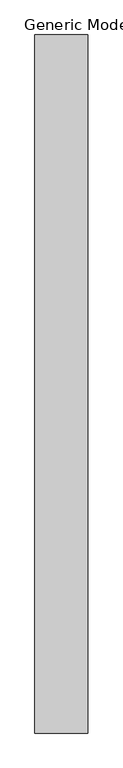
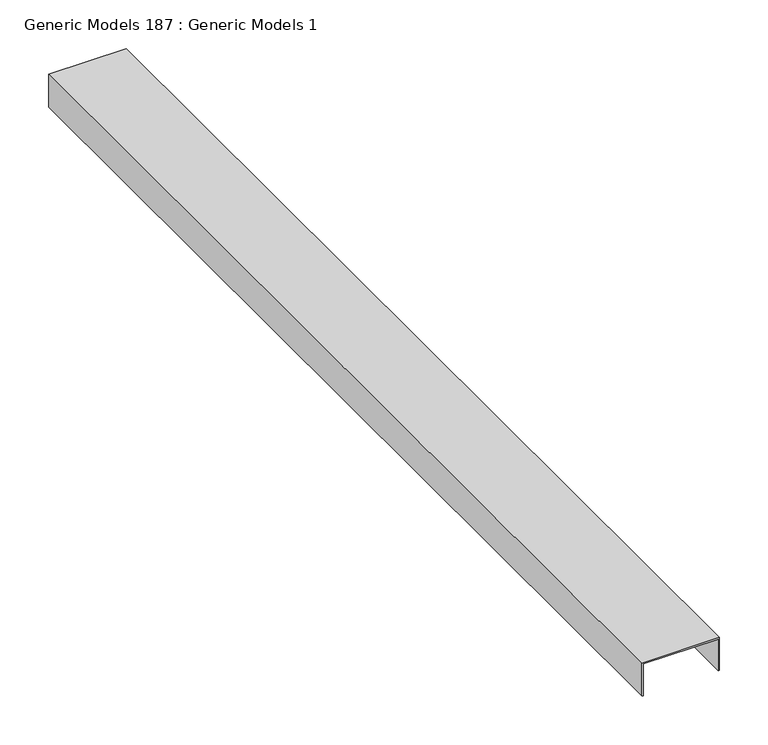
"""IFC4 building model written with IfcOpenShell, lengths in millimetres: proxy geometry, Generic Models 187 : Generic Models 1."""

import ifcopenshell
import ifcopenshell.guid

model = None  # the IFC model being written
_history = None  # IfcOwnerHistory: only IFC2X3 demands one
_inside = {}  # id of a spatial element -> (the spatial element, [elements in it])
_under = {}  # id of a project, library or spatial element -> (it, [spatial elements below it])
_declared = {}  # id of a project -> (the project, [libraries it declares])
_typed = {}  # id of a type object -> (the type object, [elements of that type])
_made_of = {}  # id of a material, layer set ... -> (it, [elements and type objects made of it])


def new_model(schema):
    """Start an empty IFC model of exactly this schema.

    Asked for "IFC4X3", IfcOpenShell would pick the latest addendum, in which some entities
    have other attributes; the version numbers below select the first issue.
    IFC2X3 requires an IfcOwnerHistory on every rooted entity: one is made here for all.
    """
    global model, _history
    if schema == "IFC4X3":
        model = ifcopenshell.file(schema_version=(4, 3, 0, 0))
    else:
        model = ifcopenshell.file(schema=schema)
    _inside.clear()
    _under.clear()
    _declared.clear()
    _typed.clear()
    _made_of.clear()
    _history = None
    if model.schema == "IFC2X3":
        org = make("IfcOrganization", Name="unknown")
        user = make(
            "IfcPersonAndOrganization",
            ThePerson=make("IfcPerson", FamilyName="unknown"),
            TheOrganization=org,
        )
        app = make(
            "IfcApplication",
            ApplicationDeveloper=org,
            Version="unknown",
            ApplicationFullName="unknown",
            ApplicationIdentifier="unknown",
        )
        _history = make(
            "IfcOwnerHistory",
            OwningUser=user,
            OwningApplication=app,
            ChangeAction="ADDED",
            CreationDate=0,
        )
    return model


def make(cls, **values):
    """One entity of the class cls with the attributes given. An attribute that is None is left unset."""
    return model.create_entity(
        cls, **{name: value for name, value in values.items() if value is not None}
    )


def rooted(cls, **values):
    """An entity with a GlobalId (a new one), such as an element, a storey or a relation."""
    return make(cls, GlobalId=ifcopenshell.guid.new(), OwnerHistory=_history, **values)


def si_unit(unit_type, name, prefix=None):
    """IfcSIUnit, for example si_unit("LENGTHUNIT", "METRE", prefix="MILLI")."""
    return make("IfcSIUnit", UnitType=unit_type, Prefix=prefix, Name=name)


def assignment(units):
    """IfcUnitAssignment: the units of a project."""
    return None if units is None else make("IfcUnitAssignment", Units=units)


def point(xyz):
    """IfcCartesianPoint."""
    return None if xyz is None else make("IfcCartesianPoint", Coordinates=xyz)


def direction(xyz):
    """IfcDirection."""
    return None if xyz is None else make("IfcDirection", DirectionRatios=xyz)


def frame(location, z_axis=None, x_axis=None):
    """IfcAxis2Placement3D, a coordinate frame: its origin and axes. An axis left out is left unset."""
    return make(
        "IfcAxis2Placement3D",
        Location=point(location),
        Axis=direction(z_axis),
        RefDirection=direction(x_axis),
    )


def origin():
    """The frame at (0, 0, 0) with its axes left unset."""
    return frame((0.0, 0.0, 0.0))


def place(relative_to, where):
    """IfcLocalPlacement: puts the frame where relative to a parent placement (None: the world)."""
    return make(
        "IfcLocalPlacement", PlacementRelTo=relative_to, RelativePlacement=where
    )


def context(
    kind, dimensions, precision=None, world=None, true_north=None, identifier=None
):
    """IfcGeometricRepresentationContext, for example the 3D "Model" context."""
    return make(
        "IfcGeometricRepresentationContext",
        ContextIdentifier=identifier,
        ContextType=kind,
        CoordinateSpaceDimension=dimensions,
        Precision=precision,
        WorldCoordinateSystem=world,
        TrueNorth=true_north,
    )


def project(units=None, contexts=None):
    """IfcProject with its units and contexts."""
    return rooted(
        "IfcProject",
        Name="project",
        RepresentationContexts=contexts,
        UnitsInContext=assignment(units),
    )


def spatial(cls, under=None, at=None, **own):
    """A site, building, storey or space (cls), placed at a placement, below another one or the project."""
    s = rooted(cls, ObjectPlacement=at, **own)
    if under is not None:
        _under.setdefault(under.id(), (under, []))[1].append(s)
    return s


def polyline(points):
    """IfcPolyline through the points."""
    return make("IfcPolyline", Points=[point(p) for p in points])


def outline(outer, holes=None, kind="AREA"):
    """IfcArbitraryClosedProfileDef: a profile drawn as a closed curve; with holes, ...WithVoids."""
    if holes is None:
        return make("IfcArbitraryClosedProfileDef", ProfileType=kind, OuterCurve=outer)
    return make(
        "IfcArbitraryProfileDefWithVoids",
        ProfileType=kind,
        OuterCurve=outer,
        InnerCurves=holes,
    )


def extrude(swept, where, along, depth):
    """IfcExtrudedAreaSolid: the profile swept, set in the frame where, extruded along a direction by depth."""
    return make(
        "IfcExtrudedAreaSolid",
        SweptArea=swept,
        Position=where,
        ExtrudedDirection=direction(along),
        Depth=depth,
    )


def shape(context_of_items, identifier, shape_type, items):
    """IfcShapeRepresentation: the items that make up one representation, for example the "Body"."""
    return make(
        "IfcShapeRepresentation",
        ContextOfItems=context_of_items,
        RepresentationIdentifier=identifier,
        RepresentationType=shape_type,
        Items=items,
    )


def source(mapping_origin, context_of_items, identifier, shape_type, items):
    """IfcRepresentationMap: a shape defined once, which mapped items show again and again."""
    return make(
        "IfcRepresentationMap",
        MappingOrigin=mapping_origin,
        MappedRepresentation=shape(context_of_items, identifier, shape_type, items),
    )


def transform(
    local_origin,
    x_axis=None,
    y_axis=None,
    z_axis=None,
    scale=None,
    scale2=None,
    scale3=None,
    uniform=True,
):
    """IfcCartesianTransformationOperator3D, or its non-uniform kind. x_axis, y_axis, z_axis: its Axis1, 2, 3."""
    if uniform:
        return make(
            "IfcCartesianTransformationOperator3D",
            Axis1=direction(x_axis),
            Axis2=direction(y_axis),
            LocalOrigin=point(local_origin),
            Scale=scale,
            Axis3=direction(z_axis),
        )
    return make(
        "IfcCartesianTransformationOperator3DnonUniform",
        Axis1=direction(x_axis),
        Axis2=direction(y_axis),
        LocalOrigin=point(local_origin),
        Scale=scale,
        Axis3=direction(z_axis),
        Scale2=scale2,
        Scale3=scale3,
    )


def mapped(mapping_source, mapping_target):
    """IfcMappedItem: shows the shape of a source again, moved by a transform."""
    return make(
        "IfcMappedItem", MappingSource=mapping_source, MappingTarget=mapping_target
    )


def made_of(thing, what):
    """Note that an element or type object is made of a material, layer set ...; save() writes the relation."""
    if what is not None:
        _made_of.setdefault(what.id(), (what, []))[1].append(thing)
    return thing


def element(
    cls,
    number,
    at=None,
    inside=None,
    cuts=None,
    type_object=None,
    material=None,
    context=None,
    identifier="Body",
    shape_type=None,
    held_by="IfcProductDefinitionShape",
    body=None,
    shapes=None,
    **own,
):
    """One element of the class cls, such as IfcWall. Its Tag is "e" and its number.

    at: its placement. inside: the storey or other place that contains it. cuts: it is an
    opening in that element (IfcRelVoidsElement). A single representation is given by context,
    identifier, shape_type and body (its items); several are given by shapes. held_by: the class
    of the entity that holds the representations. save() writes the other relations.
    """
    e = rooted(cls, Tag="e%d" % number, ObjectPlacement=at, **own)
    if body is not None:
        shapes = [shape(context, identifier, shape_type, body)]
    if shapes is not None:
        e.Representation = make(held_by, Representations=shapes)
    if inside is not None:
        _inside.setdefault(inside.id(), (inside, []))[1].append(e)
    if cuts is not None:
        rooted(
            "IfcRelVoidsElement", RelatingBuildingElement=cuts, RelatedOpeningElement=e
        )
    if type_object is not None:
        _typed.setdefault(type_object.id(), (type_object, []))[1].append(e)
    return made_of(e, material)


def aggregate(whole, parts):
    """IfcRelAggregates: a whole, such as a stair, and the parts it consists of."""
    return rooted("IfcRelAggregates", RelatingObject=whole, RelatedObjects=parts)


def save(model, path):
    """Write the relations noted so far, then the file.

    IfcRelAggregates (storeys below a building ...), IfcRelContainedInSpatialStructure (elements
    in a storey), IfcRelDefinesByType, IfcRelAssociatesMaterial and IfcRelDeclares: one each for
    every whole, place, type object, material and project.
    """
    for whole, parts in _under.values():
        aggregate(whole, parts)
    for where, things in _inside.values():
        rooted(
            "IfcRelContainedInSpatialStructure",
            RelatedElements=things,
            RelatingStructure=where,
        )
    for kind, things in _typed.values():
        rooted("IfcRelDefinesByType", RelatedObjects=things, RelatingType=kind)
    for what, things in _made_of.values():
        rooted("IfcRelAssociatesMaterial", RelatedObjects=things, RelatingMaterial=what)
    for by, libraries in _declared.values():
        rooted("IfcRelDeclares", RelatingContext=by, RelatedDefinitions=libraries)
    model.write(path)


def generic_models_187_generic_models_1_fb1cd1ca(model_context):
    return source(origin(), model_context, "Body", "SweptSolid", [
        extrude(outline(polyline([(533.0026794, 52650.4446108), (533.0026794, 52558.3696108), (491.7276794, 52558.3696108), (491.7276794, 52559.9571108), (531.4151794, 52559.9571108), (531.4151794, 52648.8571108), (491.7276794, 52648.8571108), (491.7276794, 52650.4446108), (533.0026794, 52650.4446108)])), frame((0.0, 0.0, 0.0), z_axis=(0.0, 1.0, 0.0), x_axis=(0.0, 0.0, 1.0)), (0.0, 0.0, 1.0), 1219.2),
    ])


if __name__ == "__main__":
    model = new_model("IFC4")
    model_context = context("Model", 3, world=origin())
    ifc_project = project(units=[si_unit("LENGTHUNIT", "METRE", prefix="MILLI")], contexts=[model_context])
    site = spatial("IfcSite", under=ifc_project)
    building = spatial("IfcBuilding", under=site)
    placement = place(None, origin())
    generic_models_187_generic_models_1_shape = generic_models_187_generic_models_1_fb1cd1ca(model_context)
    element("IfcBuildingElementProxy", 1, Name="Generic Models 187 : Generic Models 1", ObjectType="Generic Models 187 : Generic Models 1", at=placement, inside=building, context=model_context, shape_type="MappedRepresentation", body=[
        mapped(generic_models_187_generic_models_1_shape, transform((0.0, 0.0, 0.0), x_axis=(1.0, 0.0, 0.0), y_axis=(0.0, 1.0, 0.0), z_axis=(0.0, 0.0, 1.0))),
    ])
    save(model, "model.ifc")

# Revit data of these elements
# Element 1 (IfcBuildingElementProxy, "Generic Models 187 : Generic Models 1")
#   Materials on its faces: "DEEP LEG OF DEFLECTION TRACK (2\" MIN. DEFLECTION)"
# Materials
#   "DEEP LEG OF DEFLECTION TRACK (2\" MIN. DEFLECTION)": class "Unassigned", colour RGB 210 209 208, transparency 0, Keynote = "M05121300.02", Cost = 0
